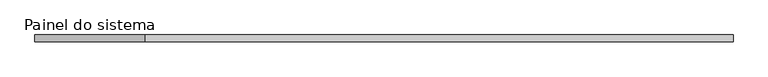
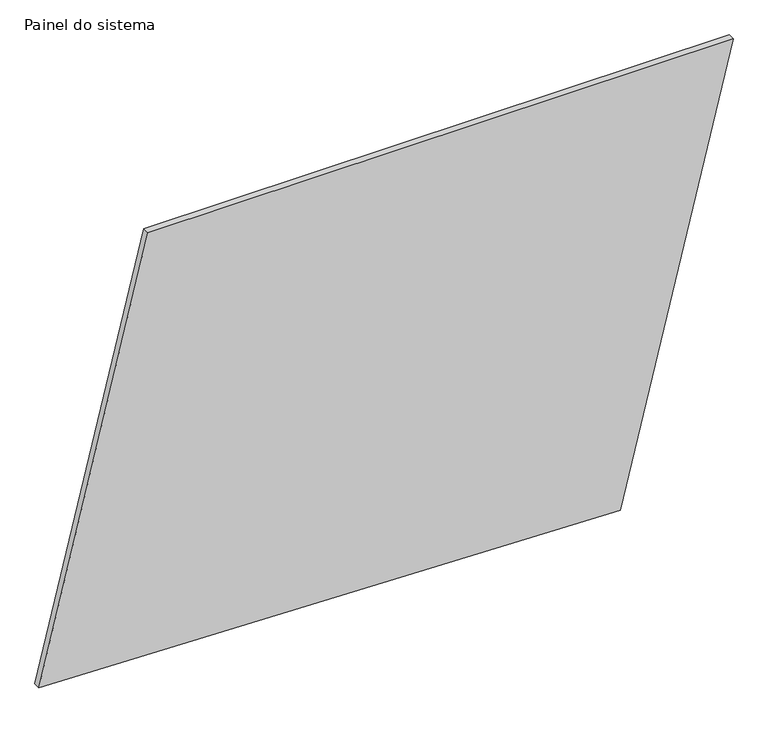
"""IFC4 building model written with IfcOpenShell, lengths in millimetres: plate geometry, Painel do sistema : Envidraçado."""

import ifcopenshell
import ifcopenshell.guid

model = None  # the IFC model being written
_history = None  # IfcOwnerHistory: only IFC2X3 demands one
_inside = {}  # id of a spatial element -> (the spatial element, [elements in it])
_under = {}  # id of a project, library or spatial element -> (it, [spatial elements below it])
_declared = {}  # id of a project -> (the project, [libraries it declares])
_typed = {}  # id of a type object -> (the type object, [elements of that type])
_made_of = {}  # id of a material, layer set ... -> (it, [elements and type objects made of it])


def new_model(schema):
    """Start an empty IFC model of exactly this schema.

    Asked for "IFC4X3", IfcOpenShell would pick the latest addendum, in which some entities
    have other attributes; the version numbers below select the first issue.
    IFC2X3 requires an IfcOwnerHistory on every rooted entity: one is made here for all.
    """
    global model, _history
    if schema == "IFC4X3":
        model = ifcopenshell.file(schema_version=(4, 3, 0, 0))
    else:
        model = ifcopenshell.file(schema=schema)
    _inside.clear()
    _under.clear()
    _declared.clear()
    _typed.clear()
    _made_of.clear()
    _history = None
    if model.schema == "IFC2X3":
        org = make("IfcOrganization", Name="unknown")
        user = make(
            "IfcPersonAndOrganization",
            ThePerson=make("IfcPerson", FamilyName="unknown"),
            TheOrganization=org,
        )
        app = make(
            "IfcApplication",
            ApplicationDeveloper=org,
            Version="unknown",
            ApplicationFullName="unknown",
            ApplicationIdentifier="unknown",
        )
        _history = make(
            "IfcOwnerHistory",
            OwningUser=user,
            OwningApplication=app,
            ChangeAction="ADDED",
            CreationDate=0,
        )
    return model


def make(cls, **values):
    """One entity of the class cls with the attributes given. An attribute that is None is left unset."""
    return model.create_entity(
        cls, **{name: value for name, value in values.items() if value is not None}
    )


def rooted(cls, **values):
    """An entity with a GlobalId (a new one), such as an element, a storey or a relation."""
    return make(cls, GlobalId=ifcopenshell.guid.new(), OwnerHistory=_history, **values)


def si_unit(unit_type, name, prefix=None):
    """IfcSIUnit, for example si_unit("LENGTHUNIT", "METRE", prefix="MILLI")."""
    return make("IfcSIUnit", UnitType=unit_type, Prefix=prefix, Name=name)


def assignment(units):
    """IfcUnitAssignment: the units of a project."""
    return None if units is None else make("IfcUnitAssignment", Units=units)


def point(xyz):
    """IfcCartesianPoint."""
    return None if xyz is None else make("IfcCartesianPoint", Coordinates=xyz)


def direction(xyz):
    """IfcDirection."""
    return None if xyz is None else make("IfcDirection", DirectionRatios=xyz)


def frame(location, z_axis=None, x_axis=None):
    """IfcAxis2Placement3D, a coordinate frame: its origin and axes. An axis left out is left unset."""
    return make(
        "IfcAxis2Placement3D",
        Location=point(location),
        Axis=direction(z_axis),
        RefDirection=direction(x_axis),
    )


def origin():
    """The frame at (0, 0, 0) with its axes left unset."""
    return frame((0.0, 0.0, 0.0))


def place(relative_to, where):
    """IfcLocalPlacement: puts the frame where relative to a parent placement (None: the world)."""
    return make(
        "IfcLocalPlacement", PlacementRelTo=relative_to, RelativePlacement=where
    )


def context(
    kind, dimensions, precision=None, world=None, true_north=None, identifier=None
):
    """IfcGeometricRepresentationContext, for example the 3D "Model" context."""
    return make(
        "IfcGeometricRepresentationContext",
        ContextIdentifier=identifier,
        ContextType=kind,
        CoordinateSpaceDimension=dimensions,
        Precision=precision,
        WorldCoordinateSystem=world,
        TrueNorth=true_north,
    )


def project(units=None, contexts=None):
    """IfcProject with its units and contexts."""
    return rooted(
        "IfcProject",
        Name="project",
        RepresentationContexts=contexts,
        UnitsInContext=assignment(units),
    )


def spatial(cls, under=None, at=None, **own):
    """A site, building, storey or space (cls), placed at a placement, below another one or the project."""
    s = rooted(cls, ObjectPlacement=at, **own)
    if under is not None:
        _under.setdefault(under.id(), (under, []))[1].append(s)
    return s


def polyline(points):
    """IfcPolyline through the points."""
    return make("IfcPolyline", Points=[point(p) for p in points])


def outline(outer, holes=None, kind="AREA"):
    """IfcArbitraryClosedProfileDef: a profile drawn as a closed curve; with holes, ...WithVoids."""
    if holes is None:
        return make("IfcArbitraryClosedProfileDef", ProfileType=kind, OuterCurve=outer)
    return make(
        "IfcArbitraryProfileDefWithVoids",
        ProfileType=kind,
        OuterCurve=outer,
        InnerCurves=holes,
    )


def extrude(swept, where, along, depth):
    """IfcExtrudedAreaSolid: the profile swept, set in the frame where, extruded along a direction by depth."""
    return make(
        "IfcExtrudedAreaSolid",
        SweptArea=swept,
        Position=where,
        ExtrudedDirection=direction(along),
        Depth=depth,
    )


def shape(context_of_items, identifier, shape_type, items):
    """IfcShapeRepresentation: the items that make up one representation, for example the "Body"."""
    return make(
        "IfcShapeRepresentation",
        ContextOfItems=context_of_items,
        RepresentationIdentifier=identifier,
        RepresentationType=shape_type,
        Items=items,
    )


def source(mapping_origin, context_of_items, identifier, shape_type, items):
    """IfcRepresentationMap: a shape defined once, which mapped items show again and again."""
    return make(
        "IfcRepresentationMap",
        MappingOrigin=mapping_origin,
        MappedRepresentation=shape(context_of_items, identifier, shape_type, items),
    )


def transform(
    local_origin,
    x_axis=None,
    y_axis=None,
    z_axis=None,
    scale=None,
    scale2=None,
    scale3=None,
    uniform=True,
):
    """IfcCartesianTransformationOperator3D, or its non-uniform kind. x_axis, y_axis, z_axis: its Axis1, 2, 3."""
    if uniform:
        return make(
            "IfcCartesianTransformationOperator3D",
            Axis1=direction(x_axis),
            Axis2=direction(y_axis),
            LocalOrigin=point(local_origin),
            Scale=scale,
            Axis3=direction(z_axis),
        )
    return make(
        "IfcCartesianTransformationOperator3DnonUniform",
        Axis1=direction(x_axis),
        Axis2=direction(y_axis),
        LocalOrigin=point(local_origin),
        Scale=scale,
        Axis3=direction(z_axis),
        Scale2=scale2,
        Scale3=scale3,
    )


def mapped(mapping_source, mapping_target):
    """IfcMappedItem: shows the shape of a source again, moved by a transform."""
    return make(
        "IfcMappedItem", MappingSource=mapping_source, MappingTarget=mapping_target
    )


def made_of(thing, what):
    """Note that an element or type object is made of a material, layer set ...; save() writes the relation."""
    if what is not None:
        _made_of.setdefault(what.id(), (what, []))[1].append(thing)
    return thing


def element(
    cls,
    number,
    at=None,
    inside=None,
    cuts=None,
    type_object=None,
    material=None,
    context=None,
    identifier="Body",
    shape_type=None,
    held_by="IfcProductDefinitionShape",
    body=None,
    shapes=None,
    **own,
):
    """One element of the class cls, such as IfcWall. Its Tag is "e" and its number.

    at: its placement. inside: the storey or other place that contains it. cuts: it is an
    opening in that element (IfcRelVoidsElement). A single representation is given by context,
    identifier, shape_type and body (its items); several are given by shapes. held_by: the class
    of the entity that holds the representations. save() writes the other relations.
    """
    e = rooted(cls, Tag="e%d" % number, ObjectPlacement=at, **own)
    if body is not None:
        shapes = [shape(context, identifier, shape_type, body)]
    if shapes is not None:
        e.Representation = make(held_by, Representations=shapes)
    if inside is not None:
        _inside.setdefault(inside.id(), (inside, []))[1].append(e)
    if cuts is not None:
        rooted(
            "IfcRelVoidsElement", RelatingBuildingElement=cuts, RelatedOpeningElement=e
        )
    if type_object is not None:
        _typed.setdefault(type_object.id(), (type_object, []))[1].append(e)
    return made_of(e, material)


def aggregate(whole, parts):
    """IfcRelAggregates: a whole, such as a stair, and the parts it consists of."""
    return rooted("IfcRelAggregates", RelatingObject=whole, RelatedObjects=parts)


def save(model, path):
    """Write the relations noted so far, then the file.

    IfcRelAggregates (storeys below a building ...), IfcRelContainedInSpatialStructure (elements
    in a storey), IfcRelDefinesByType, IfcRelAssociatesMaterial and IfcRelDeclares: one each for
    every whole, place, type object, material and project.
    """
    for whole, parts in _under.values():
        aggregate(whole, parts)
    for where, things in _inside.values():
        rooted(
            "IfcRelContainedInSpatialStructure",
            RelatedElements=things,
            RelatingStructure=where,
        )
    for kind, things in _typed.values():
        rooted("IfcRelDefinesByType", RelatedObjects=things, RelatingType=kind)
    for what, things in _made_of.values():
        rooted("IfcRelAssociatesMaterial", RelatedObjects=things, RelatingMaterial=what)
    for by, libraries in _declared.values():
        rooted("IfcRelDeclares", RelatingContext=by, RelatedDefinitions=libraries)
    model.write(path)


def painel_do_sistema_1a8f51e3(model_context):
    return source(origin(), model_context, "Body", "SweptSolid", [
        extrude(outline(polyline([(57.8498312, -1259.6186536), (0.0, 849.5639812), (1665.5325421, 1259.6186536), (1665.5325421, -863.8066291), (57.8498312, -1259.6186536)])), frame((0.0, 24.5, 0.0), z_axis=(0.0, 1.0, 0.0), x_axis=(0.0, 0.0, 1.0)), (0.0, 0.0, 1.0), 25.0),
    ])


if __name__ == "__main__":
    model = new_model("IFC4")
    model_context = context("Model", 3, world=origin())
    ifc_project = project(units=[si_unit("LENGTHUNIT", "METRE", prefix="MILLI")], contexts=[model_context])
    site = spatial("IfcSite", under=ifc_project)
    building = spatial("IfcBuilding", under=site)
    placement = place(None, origin())
    painel_do_sistema_shape = painel_do_sistema_1a8f51e3(model_context)
    element("IfcPlate", 1, ObjectType="Painel do sistema : Envidraçado", at=placement, inside=building, context=model_context, shape_type="MappedRepresentation", body=[
        mapped(painel_do_sistema_shape, transform((0.0, 0.0, 0.0), x_axis=(1.0, 0.0, 0.0), y_axis=(0.0, 1.0, 0.0), z_axis=(0.0, 0.0, 1.0))),
    ])
    save(model, "model.ifc")

# Revit data of these elements
# Type "Painel do sistema : Envidraçado"
#   Construction Type Id = "GSP4R"
#   Analytic Construction = "Vidraça única Pilkington 1/8 pol"
#   Visual Light Transmittance = 0.9
#   Solar Heat Gain Coefficient = 0.86
#   Heat Transfer Coefficient (U) = 6.7069 W/(m²·K)
# Element 1 (IfcPlate, "Painel do sistema : Envidraçado")
#   Materials on its faces: "Vidro"
# Materials
#   "Vidro": class "Vidro", colour RGB 0 128 192, transparency 0.9, Description = "Vidro de sílica", Cost = 0
